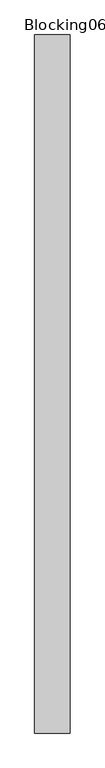
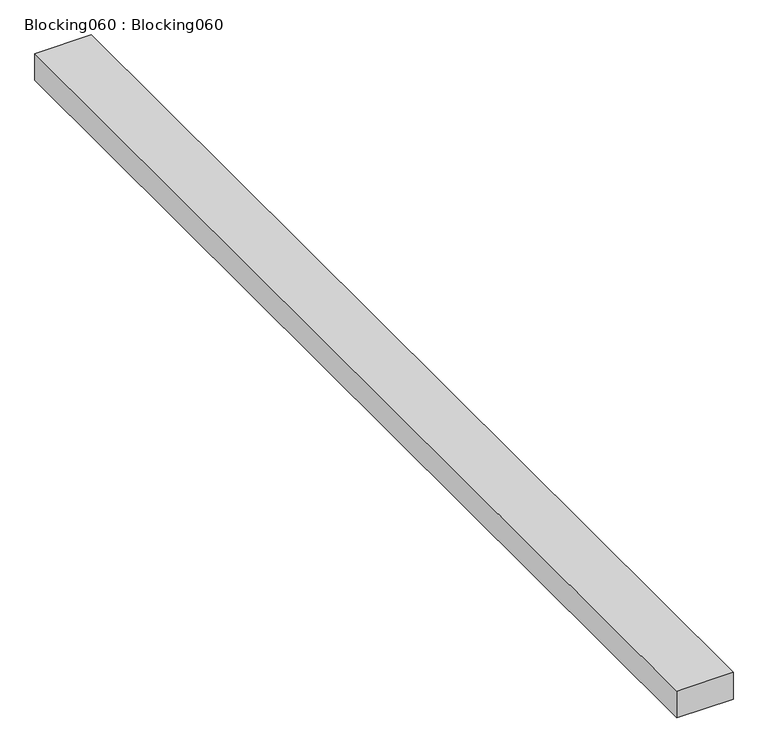
"""IFC4 building model written with IfcOpenShell, lengths in millimetres: proxy geometry, Blocking060 : Blocking060."""

from ifc_helpers import new_model, si_unit, frame, origin, place, context, project, spatial, polyline, outline, extrude, source, transform, mapped, element, save


def blocking060_blocking060_221e796e(model_context):
    return source(origin(), model_context, "Body", "SweptSolid", [
        extrude(outline(polyline([(-7121.5276325, 7982.1531721), (-7223.1276325, 7982.1531721), (-7223.1276325, 9982.1531721), (-7121.5276325, 9982.1531721), (-7121.5276325, 7982.1531721)])), frame((0.0, 0.0, 40055.5460083), z_axis=(0.0, 0.0, 1.0), x_axis=(1.0, 0.0, 0.0)), (0.0, 0.0, 1.0), 50.8),
    ])


if __name__ == "__main__":
    model = new_model("IFC4")
    model_context = context("Model", 3, world=origin())
    ifc_project = project(units=[si_unit("LENGTHUNIT", "METRE", prefix="MILLI")], contexts=[model_context])
    site = spatial("IfcSite", under=ifc_project)
    building = spatial("IfcBuilding", under=site)
    placement = place(None, origin())
    blocking060_blocking060_shape = blocking060_blocking060_221e796e(model_context)
    element("IfcBuildingElementProxy", 1, Name="Blocking060 : Blocking060", ObjectType="Blocking060 : Blocking060", at=placement, inside=building, context=model_context, shape_type="MappedRepresentation", body=[
        mapped(blocking060_blocking060_shape, transform((0.0, 0.0, 0.0), x_axis=(1.0, 0.0, 0.0), y_axis=(0.0, 1.0, 0.0), z_axis=(0.0, 0.0, 1.0))),
    ])
    save(model, "model.ifc")

# Revit data of these elements
# Type "Blocking060 : Blocking060"
#   NameOverride = "Blocking060"
# Element 1 (IfcBuildingElementProxy, "Blocking060 : Blocking060")
#   Materials on its faces: "WOOD BLOCKING AS REQUIRED"
# Materials
#   "WOOD BLOCKING AS REQUIRED": class "Unassigned", colour RGB 166 124 85, transparency 0, Cost = 0
